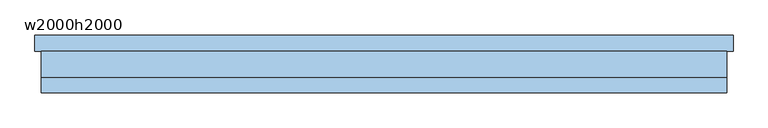
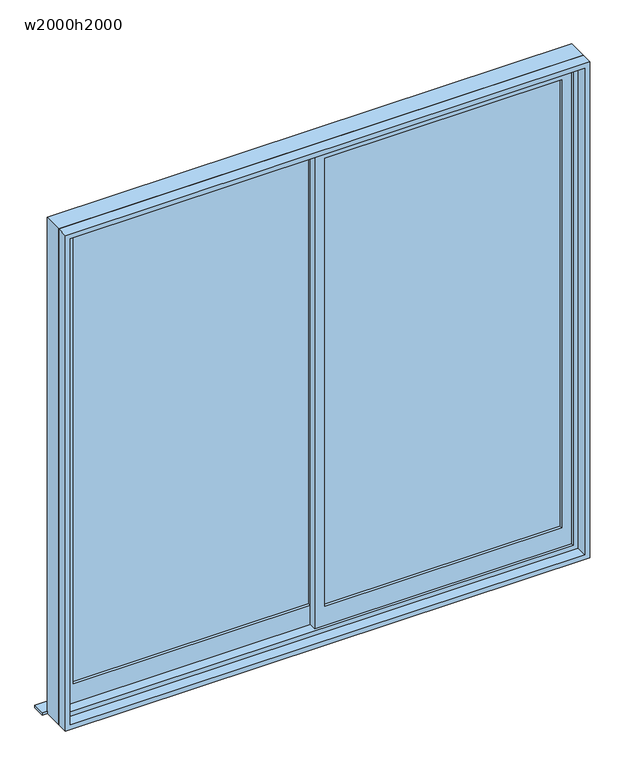
"""IFC4 building model written with IfcOpenShell, lengths in millimetres: window geometry, 引違い掃出窓_2枚 : w2000h2000."""

import ifcopenshell
import ifcopenshell.guid

model = None  # the IFC model being written
_history = None  # IfcOwnerHistory: only IFC2X3 demands one
_inside = {}  # id of a spatial element -> (the spatial element, [elements in it])
_under = {}  # id of a project, library or spatial element -> (it, [spatial elements below it])
_declared = {}  # id of a project -> (the project, [libraries it declares])
_typed = {}  # id of a type object -> (the type object, [elements of that type])
_made_of = {}  # id of a material, layer set ... -> (it, [elements and type objects made of it])


def new_model(schema):
    """Start an empty IFC model of exactly this schema.

    Asked for "IFC4X3", IfcOpenShell would pick the latest addendum, in which some entities
    have other attributes; the version numbers below select the first issue.
    IFC2X3 requires an IfcOwnerHistory on every rooted entity: one is made here for all.
    """
    global model, _history
    if schema == "IFC4X3":
        model = ifcopenshell.file(schema_version=(4, 3, 0, 0))
    else:
        model = ifcopenshell.file(schema=schema)
    _inside.clear()
    _under.clear()
    _declared.clear()
    _typed.clear()
    _made_of.clear()
    _history = None
    if model.schema == "IFC2X3":
        org = make("IfcOrganization", Name="unknown")
        user = make(
            "IfcPersonAndOrganization",
            ThePerson=make("IfcPerson", FamilyName="unknown"),
            TheOrganization=org,
        )
        app = make(
            "IfcApplication",
            ApplicationDeveloper=org,
            Version="unknown",
            ApplicationFullName="unknown",
            ApplicationIdentifier="unknown",
        )
        _history = make(
            "IfcOwnerHistory",
            OwningUser=user,
            OwningApplication=app,
            ChangeAction="ADDED",
            CreationDate=0,
        )
    return model


def make(cls, **values):
    """One entity of the class cls with the attributes given. An attribute that is None is left unset."""
    return model.create_entity(
        cls, **{name: value for name, value in values.items() if value is not None}
    )


def rooted(cls, **values):
    """An entity with a GlobalId (a new one), such as an element, a storey or a relation."""
    return make(cls, GlobalId=ifcopenshell.guid.new(), OwnerHistory=_history, **values)


def si_unit(unit_type, name, prefix=None):
    """IfcSIUnit, for example si_unit("LENGTHUNIT", "METRE", prefix="MILLI")."""
    return make("IfcSIUnit", UnitType=unit_type, Prefix=prefix, Name=name)


def assignment(units):
    """IfcUnitAssignment: the units of a project."""
    return None if units is None else make("IfcUnitAssignment", Units=units)


def point(xyz):
    """IfcCartesianPoint."""
    return None if xyz is None else make("IfcCartesianPoint", Coordinates=xyz)


def direction(xyz):
    """IfcDirection."""
    return None if xyz is None else make("IfcDirection", DirectionRatios=xyz)


def frame(location, z_axis=None, x_axis=None):
    """IfcAxis2Placement3D, a coordinate frame: its origin and axes. An axis left out is left unset."""
    return make(
        "IfcAxis2Placement3D",
        Location=point(location),
        Axis=direction(z_axis),
        RefDirection=direction(x_axis),
    )


def origin():
    """The frame at (0, 0, 0) with its axes left unset."""
    return frame((0.0, 0.0, 0.0))


def place(relative_to, where):
    """IfcLocalPlacement: puts the frame where relative to a parent placement (None: the world)."""
    return make(
        "IfcLocalPlacement", PlacementRelTo=relative_to, RelativePlacement=where
    )


def context(
    kind, dimensions, precision=None, world=None, true_north=None, identifier=None
):
    """IfcGeometricRepresentationContext, for example the 3D "Model" context."""
    return make(
        "IfcGeometricRepresentationContext",
        ContextIdentifier=identifier,
        ContextType=kind,
        CoordinateSpaceDimension=dimensions,
        Precision=precision,
        WorldCoordinateSystem=world,
        TrueNorth=true_north,
    )


def project(units=None, contexts=None):
    """IfcProject with its units and contexts."""
    return rooted(
        "IfcProject",
        Name="project",
        RepresentationContexts=contexts,
        UnitsInContext=assignment(units),
    )


def spatial(cls, under=None, at=None, **own):
    """A site, building, storey or space (cls), placed at a placement, below another one or the project."""
    s = rooted(cls, ObjectPlacement=at, **own)
    if under is not None:
        _under.setdefault(under.id(), (under, []))[1].append(s)
    return s


def polyline(points):
    """IfcPolyline through the points."""
    return make("IfcPolyline", Points=[point(p) for p in points])


def outline(outer, holes=None, kind="AREA"):
    """IfcArbitraryClosedProfileDef: a profile drawn as a closed curve; with holes, ...WithVoids."""
    if holes is None:
        return make("IfcArbitraryClosedProfileDef", ProfileType=kind, OuterCurve=outer)
    return make(
        "IfcArbitraryProfileDefWithVoids",
        ProfileType=kind,
        OuterCurve=outer,
        InnerCurves=holes,
    )


def extrude(swept, where, along, depth):
    """IfcExtrudedAreaSolid: the profile swept, set in the frame where, extruded along a direction by depth."""
    return make(
        "IfcExtrudedAreaSolid",
        SweptArea=swept,
        Position=where,
        ExtrudedDirection=direction(along),
        Depth=depth,
    )


def shape(context_of_items, identifier, shape_type, items):
    """IfcShapeRepresentation: the items that make up one representation, for example the "Body"."""
    return make(
        "IfcShapeRepresentation",
        ContextOfItems=context_of_items,
        RepresentationIdentifier=identifier,
        RepresentationType=shape_type,
        Items=items,
    )


def source(mapping_origin, context_of_items, identifier, shape_type, items):
    """IfcRepresentationMap: a shape defined once, which mapped items show again and again."""
    return make(
        "IfcRepresentationMap",
        MappingOrigin=mapping_origin,
        MappedRepresentation=shape(context_of_items, identifier, shape_type, items),
    )


def transform(
    local_origin,
    x_axis=None,
    y_axis=None,
    z_axis=None,
    scale=None,
    scale2=None,
    scale3=None,
    uniform=True,
):
    """IfcCartesianTransformationOperator3D, or its non-uniform kind. x_axis, y_axis, z_axis: its Axis1, 2, 3."""
    if uniform:
        return make(
            "IfcCartesianTransformationOperator3D",
            Axis1=direction(x_axis),
            Axis2=direction(y_axis),
            LocalOrigin=point(local_origin),
            Scale=scale,
            Axis3=direction(z_axis),
        )
    return make(
        "IfcCartesianTransformationOperator3DnonUniform",
        Axis1=direction(x_axis),
        Axis2=direction(y_axis),
        LocalOrigin=point(local_origin),
        Scale=scale,
        Axis3=direction(z_axis),
        Scale2=scale2,
        Scale3=scale3,
    )


def mapped(mapping_source, mapping_target):
    """IfcMappedItem: shows the shape of a source again, moved by a transform."""
    return make(
        "IfcMappedItem", MappingSource=mapping_source, MappingTarget=mapping_target
    )


def made_of(thing, what):
    """Note that an element or type object is made of a material, layer set ...; save() writes the relation."""
    if what is not None:
        _made_of.setdefault(what.id(), (what, []))[1].append(thing)
    return thing


def element(
    cls,
    number,
    at=None,
    inside=None,
    cuts=None,
    type_object=None,
    material=None,
    context=None,
    identifier="Body",
    shape_type=None,
    held_by="IfcProductDefinitionShape",
    body=None,
    shapes=None,
    **own,
):
    """One element of the class cls, such as IfcWall. Its Tag is "e" and its number.

    at: its placement. inside: the storey or other place that contains it. cuts: it is an
    opening in that element (IfcRelVoidsElement). A single representation is given by context,
    identifier, shape_type and body (its items); several are given by shapes. held_by: the class
    of the entity that holds the representations. save() writes the other relations.
    """
    e = rooted(cls, Tag="e%d" % number, ObjectPlacement=at, **own)
    if body is not None:
        shapes = [shape(context, identifier, shape_type, body)]
    if shapes is not None:
        e.Representation = make(held_by, Representations=shapes)
    if inside is not None:
        _inside.setdefault(inside.id(), (inside, []))[1].append(e)
    if cuts is not None:
        rooted(
            "IfcRelVoidsElement", RelatingBuildingElement=cuts, RelatedOpeningElement=e
        )
    if type_object is not None:
        _typed.setdefault(type_object.id(), (type_object, []))[1].append(e)
    return made_of(e, material)


def aggregate(whole, parts):
    """IfcRelAggregates: a whole, such as a stair, and the parts it consists of."""
    return rooted("IfcRelAggregates", RelatingObject=whole, RelatedObjects=parts)


def save(model, path):
    """Write the relations noted so far, then the file.

    IfcRelAggregates (storeys below a building ...), IfcRelContainedInSpatialStructure (elements
    in a storey), IfcRelDefinesByType, IfcRelAssociatesMaterial and IfcRelDeclares: one each for
    every whole, place, type object, material and project.
    """
    for whole, parts in _under.values():
        aggregate(whole, parts)
    for where, things in _inside.values():
        rooted(
            "IfcRelContainedInSpatialStructure",
            RelatedElements=things,
            RelatingStructure=where,
        )
    for kind, things in _typed.values():
        rooted("IfcRelDefinesByType", RelatedObjects=things, RelatingType=kind)
    for what, things in _made_of.values():
        rooted("IfcRelAssociatesMaterial", RelatedObjects=things, RelatingMaterial=what)
    for by, libraries in _declared.values():
        rooted("IfcRelDeclares", RelatingContext=by, RelatedDefinitions=libraries)
    model.write(path)


def w2000h2000_8e7da428(model_context):
    return source(origin(), model_context, "Body", "SweptSolid", [
        extrude(outline(polyline([(-20.0, 12.5), (-960.0, 12.5), (-960.0, 17.5), (-20.0, 17.5), (-20.0, 12.5)])), frame((0.0, 0.0, 80.0), z_axis=(0.0, 0.0, 1.0), x_axis=(1.0, 0.0, 0.0)), (0.0, 0.0, 1.0), 1880.0),
        extrude(outline(polyline([(960.0, -17.5), (20.0, -17.5), (20.0, -12.5), (960.0, -12.5), (960.0, -17.5)])), frame((0.0, 0.0, 80.0), z_axis=(0.0, 0.0, 1.0), x_axis=(1.0, 0.0, 0.0)), (0.0, 0.0, 1.0), 1880.0),
        extrude(outline(polyline([(2000.0, -20.0), (0.0, -20.0), (0.0, 1000.0), (2000.0, 1000.0), (2000.0, -20.0)]), holes=[polyline([(80.0, 960.0), (80.0, 20.0), (1960.0, 20.0), (1960.0, 960.0), (80.0, 960.0)])]), frame((0.0, -30.0, 0.0), z_axis=(0.0, 1.0, 0.0), x_axis=(0.0, 0.0, 1.0)), (0.0, 0.0, 1.0), 30.0),
        extrude(outline(polyline([(2000.0, -1000.0), (0.0, -1000.0), (0.0, 20.0), (2000.0, 20.0), (2000.0, -1000.0)]), holes=[polyline([(80.0, -20.0), (80.0, -960.0), (1960.0, -960.0), (1960.0, -20.0), (80.0, -20.0)])]), frame((0.0, 0.0, 0.0), z_axis=(0.0, 1.0, 0.0), x_axis=(0.0, 0.0, 1.0)), (0.0, 0.0, 1.0), 30.0),
        extrude(outline(polyline([(1060.0, 90.0), (1060.0, 40.0), (-1060.0, 40.0), (-1060.0, 90.0), (1060.0, 90.0)])), frame((0.0, 0.0, -40.0), z_axis=(0.0, 0.0, 1.0), x_axis=(1.0, 0.0, 0.0)), (0.0, 0.0, 1.0), 10.0),
        extrude(outline(polyline([(2040.0, 1040.0), (2040.0, -1040.0), (-40.0, -1040.0), (-40.0, 1040.0), (2040.0, 1040.0)]), holes=[polyline([(-20.0, -1020.0), (2020.0, -1020.0), (2020.0, 1020.0), (-20.0, 1020.0), (-20.0, -1020.0)])]), frame((0.0, -85.0, 0.0), z_axis=(0.0, 1.0, 0.0), x_axis=(0.0, 0.0, 1.0)), (0.0, 0.0, 1.0), 45.0),
        extrude(outline(polyline([(2040.0, -1040.0), (-40.0, -1040.0), (-40.0, 1040.0), (2040.0, 1040.0), (2040.0, -1040.0)]), holes=[polyline([(2000.0, 1000.0), (0.0, 1000.0), (0.0, -1000.0), (2000.0, -1000.0), (2000.0, 1000.0)])]), frame((0.0, -40.0, 0.0), z_axis=(0.0, 1.0, 0.0), x_axis=(0.0, 0.0, 1.0)), (0.0, 0.0, 1.0), 80.0),
    ])


if __name__ == "__main__":
    model = new_model("IFC4")
    model_context = context("Model", 3, world=origin())
    ifc_project = project(units=[si_unit("LENGTHUNIT", "METRE", prefix="MILLI")], contexts=[model_context])
    site = spatial("IfcSite", under=ifc_project)
    building = spatial("IfcBuilding", under=site)
    placement = place(None, origin())
    w2000h2000_shape = w2000h2000_8e7da428(model_context)
    element("IfcWindow", 1, ObjectType="引違い掃出窓_2枚 : w2000h2000", at=placement, inside=building, context=model_context, shape_type="MappedRepresentation", body=[
        mapped(w2000h2000_shape, transform((0.0, 0.0, 0.0), x_axis=(1.0, 0.0, 0.0), y_axis=(0.0, 1.0, 0.0), z_axis=(0.0, 0.0, 1.0))),
    ])
    save(model, "model.ifc")

# Revit data of these elements
# Type "引違い掃出窓_2枚 : w2000h2000"
#   Construction Type Id = "GSP4R"
#   Analytic Construction = "1/8 インチ ピルキントン一重ガラス"
#   Type Mark = "70"
#   Operation = "ダブル パネル縦"
#   Keynote = "08520.R1"
#   Visual Light Transmittance = 0.9
#   Solar Heat Gain Coefficient = 0.86
#   Heat Transfer Coefficient (U) = 6.7069 W/(m²·K)
#   Height = 2000 mm
#   既定の腰高 = 0 mm
#   Width = 2000 mm
#   額縁見附 = 20 mm
#   額縁ちり = 10 mm
#   サッシ見附 = 40 mm
#   サッシの幅 = 80 mm
#   サッシ額縁 [instance default] = none
#   サッシ本体 [instance default] = none
#   サッシガラス [instance default] = ガラス - 透明
#   Manufacturer = ""
#   Wall Closure = (empty or 0)
#   Model = ""
#   Type Comments = ""
#   Assembly Code = ""
# Element 1 (IfcWindow, "引違い掃出窓_2枚 : w2000h2000")
#   Materials on its faces: "ガラス - 透明"
# Materials
#   "ガラス - 透明": class "ガラス", colour RGB 0 128 192, transparency 0.9, Cost = 0
